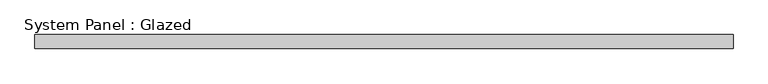
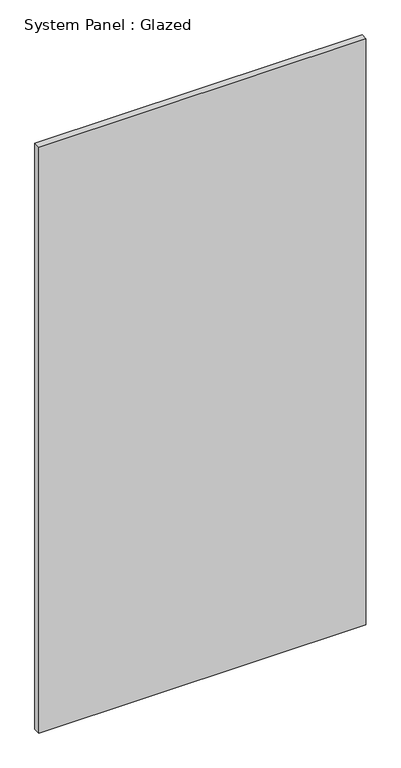
"""IFC4 building model written with IfcOpenShell, lengths in millimetres: plate geometry, System Panel : Glazed."""

from ifc_helpers import new_model, si_unit, origin, origin_with_axes, place, context, project, spatial, polyline, outline, extrude, source, transform, mapped, element, save


def system_panel_glazed_0ac89df4(model_context):
    return source(origin(), model_context, "Body", "SweptSolid", [
        extrude(outline(polyline([(620.5541356, 24.5), (-620.5541356, 24.5), (-620.5541356, 49.5), (620.5541356, 49.5), (620.5541356, 24.5)])), origin_with_axes(), (0.0, 0.0, 1.0), 2350.0),
    ])


if __name__ == "__main__":
    model = new_model("IFC4")
    model_context = context("Model", 3, world=origin())
    ifc_project = project(units=[si_unit("LENGTHUNIT", "METRE", prefix="MILLI")], contexts=[model_context])
    site = spatial("IfcSite", under=ifc_project)
    building = spatial("IfcBuilding", under=site)
    placement = place(None, origin())
    system_panel_glazed_shape = system_panel_glazed_0ac89df4(model_context)
    element("IfcPlate", 1, ObjectType="System Panel : Glazed", at=placement, inside=building, context=model_context, shape_type="MappedRepresentation", body=[
        mapped(system_panel_glazed_shape, transform((0.0, 0.0, 0.0), x_axis=(1.0, 0.0, 0.0), y_axis=(0.0, 1.0, 0.0), z_axis=(0.0, 0.0, 1.0))),
    ])
    save(model, "model.ifc")

# Revit data of these elements
# Type "System Panel : Glazed"
#   Construction Type Id = "GSP4R"
#   Analytic Construction = "1/8 in Pilkington single glazing"
#   Visual Light Transmittance = 0.9
#   Solar Heat Gain Coefficient = 0.86
#   Heat Transfer Coefficient (U) = 6.7069 W/(m²·K)
#   Define Thermal Properties by = 1
# Element 1 (IfcPlate, "System Panel : Glazed")
#   Materials on its faces: "Glass"
# Materials
#   "Glass": class "Glass", colour RGB 0 128 192, transparency 0.9, Description = "Soda Lime Glass", Cost = 0
